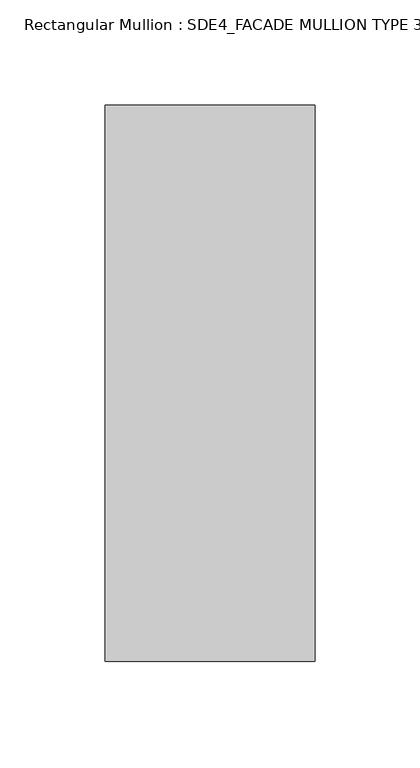
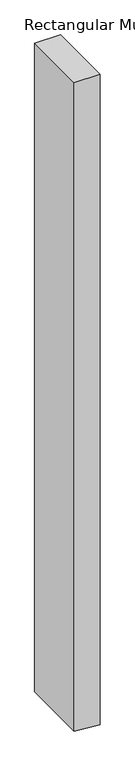
"""IFC4 building model written with IfcOpenShell, lengths in millimetres: member geometry, Rectangular Mullion : SDE4_FACADE MULLION TYPE 3."""

from ifc_helpers import new_model, si_unit, frame, origin, place, context, project, spatial, polyline, outline, extrude, source, transform, mapped, element, save


def rectangular_mullion_sde4_facade_mullion_type_3_f3c8869b(model_context):
    return source(origin(), model_context, "Body", "SweptSolid", [
        extrude(outline(polyline([(0.0, 50.0), (0.0, -50.0), (-2652.2255483, -50.0), (-2656.2916274, 3.056508), (-2659.8892247, 50.0), (0.0, 50.0)])), frame((0.0, -132.5, 0.0), z_axis=(0.0, 1.0, 0.0), x_axis=(0.0, 0.0, 1.0)), (0.0, 0.0, 1.0), 265.0),
    ])


if __name__ == "__main__":
    model = new_model("IFC4")
    model_context = context("Model", 3, world=origin())
    ifc_project = project(units=[si_unit("LENGTHUNIT", "METRE", prefix="MILLI")], contexts=[model_context])
    site = spatial("IfcSite", under=ifc_project)
    building = spatial("IfcBuilding", under=site)
    placement = place(None, origin())
    rectangular_mullion_sde4_facade_mullion_type_3_shape = rectangular_mullion_sde4_facade_mullion_type_3_f3c8869b(model_context)
    element("IfcMember", 1, ObjectType="Rectangular Mullion : SDE4_FACADE MULLION TYPE 3", at=placement, inside=building, context=model_context, shape_type="MappedRepresentation", body=[
        mapped(rectangular_mullion_sde4_facade_mullion_type_3_shape, transform((0.0, 0.0, 0.0), x_axis=(1.0, 0.0, 0.0), y_axis=(0.0, 1.0, 0.0), z_axis=(0.0, 0.0, 1.0))),
    ])
    save(model, "model.ifc")

# Revit data of these elements
# Type "Rectangular Mullion : SDE4_FACADE MULLION TYPE 3"
#   built-in parameter 1007322 = 0.869423 (stored number, unit not read)
#   built-in parameter 1007321 = 0.164042 (stored number, unit not read)
#   built-in parameter 1007320 = 0.164042 (stored number, unit not read)
